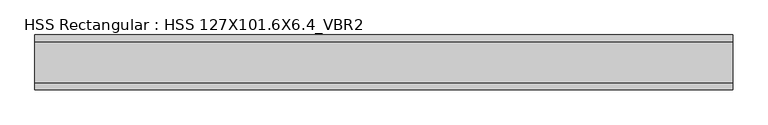
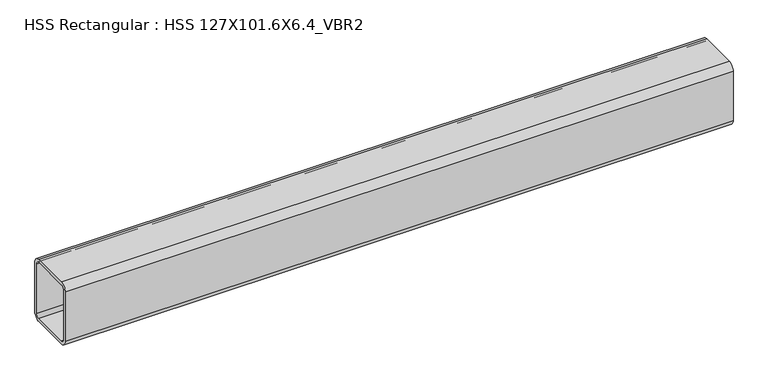
"""IFC4 building model written with IfcOpenShell, lengths in millimetres: member geometry, HSS Rectangular : HSS 127X101.6X6.4_VBR2."""

from ifc_helpers import new_model, si_unit, point, frame, frame_2d, origin, place, context, project, spatial, polyline, circle_curve, trimmed, segment, composite_curve, outline, extrude, source, transform, mapped, element, save


def hss_rectangular_hss_127x101_6x6_4_vbr2_17d18ffa(model_context):
    return source(origin(), model_context, "Body", "SweptSolid", [
        extrude(outline(composite_curve([segment(polyline([(50.8, 50.8), (50.8, -50.8)]), True, "CONTINUOUS"), segment(trimmed(circle_curve(frame_2d((38.1, -50.8)), 12.7), [point((50.8, -50.8))], [point((38.1, -63.5))], False, "CARTESIAN"), True, "CONTINUOUS"), segment(polyline([(38.1, -63.5), (-38.1, -63.5)]), True, "CONTINUOUS"), segment(trimmed(circle_curve(frame_2d((-38.1, -50.8)), 12.7), [point((-38.1, -63.5))], [point((-50.8, -50.8))], False, "CARTESIAN"), True, "CONTINUOUS"), segment(polyline([(-50.8, -50.8), (-50.8, 50.8)]), True, "CONTINUOUS"), segment(trimmed(circle_curve(frame_2d((-38.1, 50.8)), 12.7), [point((-50.8, 50.8))], [point((-38.1, 63.5))], False, "CARTESIAN"), True, "CONTINUOUS"), segment(polyline([(-38.1, 63.5), (38.1, 63.5)]), True, "CONTINUOUS"), segment(trimmed(circle_curve(frame_2d((38.1, 50.8)), 12.7), [point((38.1, 63.5))], [point((50.8, 50.8))], False, "CARTESIAN"), True, "CONTINUOUS")], self_intersect=False), holes=[composite_curve([segment(trimmed(circle_curve(frame_2d((-38.1, 50.8)), 6.35), [point((-38.1, 57.15))], [point((-44.45, 50.8))], True, "CARTESIAN"), True, "CONTINUOUS"), segment(polyline([(-44.45, 50.8), (-44.45, -50.8)]), True, "CONTINUOUS"), segment(trimmed(circle_curve(frame_2d((-38.1, -50.8)), 6.35), [point((-44.45, -50.8))], [point((-38.1, -57.15))], True, "CARTESIAN"), True, "CONTINUOUS"), segment(polyline([(-38.1, -57.15), (38.1, -57.15)]), True, "CONTINUOUS"), segment(trimmed(circle_curve(frame_2d((38.1, -50.8)), 6.35), [point((38.1, -57.15))], [point((44.45, -50.8))], True, "CARTESIAN"), True, "CONTINUOUS"), segment(polyline([(44.45, -50.8), (44.45, 50.8)]), True, "CONTINUOUS"), segment(trimmed(circle_curve(frame_2d((38.1, 50.8)), 6.35), [point((44.45, 50.8))], [point((38.1, 57.15))], True, "CARTESIAN"), True, "CONTINUOUS"), segment(polyline([(38.1, 57.15), (-38.1, 57.15)]), True, "CONTINUOUS")], self_intersect=False)]), frame((-663.9943334, 0.0, 0.0), z_axis=(1.0, 0.0, 0.0), x_axis=(0.0, 1.0, 0.0)), (0.0, 0.0, 1.0), 1293.7875462),
    ])


if __name__ == "__main__":
    model = new_model("IFC4")
    model_context = context("Model", 3, world=origin())
    ifc_project = project(units=[si_unit("LENGTHUNIT", "METRE", prefix="MILLI")], contexts=[model_context])
    site = spatial("IfcSite", under=ifc_project)
    building = spatial("IfcBuilding", under=site)
    placement = place(None, origin())
    hss_rectangular_hss_127x101_6x6_4_vbr2_shape = hss_rectangular_hss_127x101_6x6_4_vbr2_17d18ffa(model_context)
    element("IfcMember", 1, ObjectType="HSS Rectangular : HSS 127X101.6X6.4_VBR2", at=placement, inside=building, context=model_context, shape_type="MappedRepresentation", body=[
        mapped(hss_rectangular_hss_127x101_6x6_4_vbr2_shape, transform((0.0, 0.0, 0.0), x_axis=(1.0, 0.0, 0.0), y_axis=(0.0, 1.0, 0.0), z_axis=(0.0, 0.0, 1.0))),
    ])
    save(model, "model.ifc")

# Revit data of these elements
# Type "HSS Rectangular : HSS 127X101.6X6.4_VBR2"
#   Section Name Key = "HSS5X4X1/4"
#   Assembly Code = "B10"
#   Width = 10.16 cm
#   Wall Nominal Thickness = 0.635 cm
#   Wall Design Thickness = 0.5918 cm
#   Torsional Moment of Inertia = 749.217 cm⁴
#   Torsional Modulus = 136.34 cm³
#   Section Area = 24.7741 cm²
#   Plastic Modulus weak axis = 91.2759 cm³
#   Plastic Modulus strong axis = 106.352 cm³
#   Perimeter = 0.435254 m²/m
#   Outer Fillet = 1.27 cm
#   Nominal Weight = 20.7004 kgf/m
#   Moment of Inertia weak axis = 393.755 cm⁴
#   Moment of Inertia strong axis = 557.75 cm⁴
#   Inner Fillet = 0.635 cm
#   Height = 12.7 cm
#   Elastic Modulus weak axis = 77.5108 cm³
#   Elastic Modulus strong axis = 87.6708 cm³
#   Centroid Vertical = 6.35 cm
#   Centroid Horizontal = 5.08 cm
#   Length [instance default] = 1524 mm
#   Structural Material [instance default] = Steel ASTM A500, Grade C, Rectangular and Square
#   Principal Axes Angle = 0
# Element 1 (IfcMember, "HSS Rectangular : HSS 127X101.6X6.4_VBR2")
#   Materials on its faces: "Steel ASTM A500, Grade C, Rectangular and Square"
# Materials
#   "Steel ASTM A500, Grade C, Rectangular and Square": class "Metal", colour RGB 120 120 120, transparency 0, Description = "Carbon steel", Cost = 0
